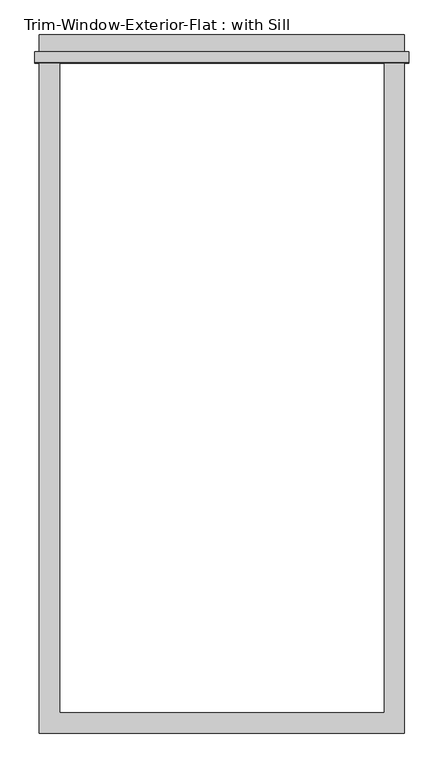
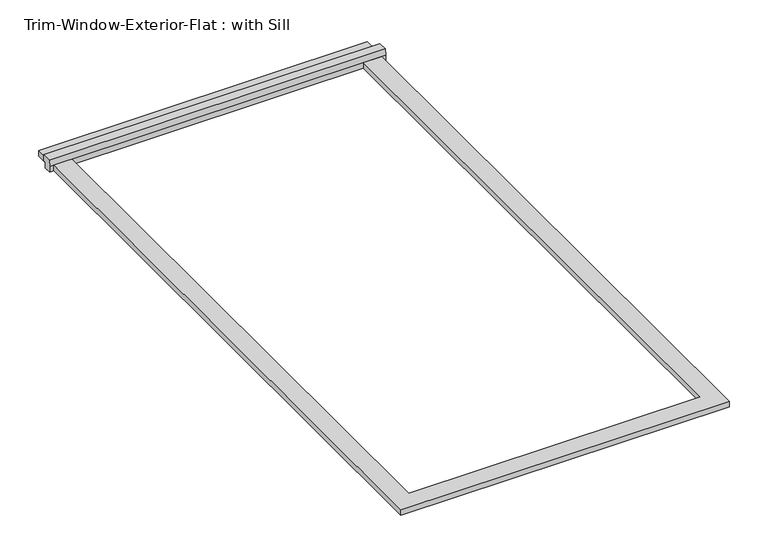
"""IFC4 building model written with IfcOpenShell, lengths in millimetres: proxy geometry, Trim-Window-Exterior-Flat : with Sill."""

from ifc_helpers import new_model, si_unit, frame, origin, origin_with_axes, place, context, project, spatial, polyline, outline, extrude, source, transform, mapped, element, save


def trim_window_exterior_flat_with_sill_0eb976c3(model_context):
    return source(origin(), model_context, "Body", "SweptSolid", [
        extrude(outline(polyline([(514.35, 1850.9823709), (-514.35, 1850.9823709), (-514.35, 1908.1323709), (514.35, 1908.1323709), (514.35, 1850.9823709)])), origin_with_axes(), (0.0, 0.0, 1.0), 19.05),
        extrude(outline(polyline([(1860.55, 38.1), (1860.55, 19.05), (1850.9823709, 19.05), (1850.9823709, 0.0), (1828.8, 0.0), (1828.8, 19.05), (1831.2580645, 38.1), (1860.55, 38.1)])), frame((-527.05, 0.0, 0.0), z_axis=(1.0, 0.0, 0.0), x_axis=(0.0, 1.0, 0.0)), (0.0, 0.0, 1.0), 1054.1),
        extrude(outline(polyline([(-514.35, -57.15), (-514.35, 1828.8), (-457.2, 1828.8), (-457.2, 0.0), (457.2, 0.0), (457.2, 1828.8), (514.35, 1828.8), (514.35, -57.15), (-514.35, -57.15)])), origin_with_axes(), (0.0, 0.0, 1.0), 19.05),
    ])


if __name__ == "__main__":
    model = new_model("IFC4")
    model_context = context("Model", 3, world=origin())
    ifc_project = project(units=[si_unit("LENGTHUNIT", "METRE", prefix="MILLI")], contexts=[model_context])
    site = spatial("IfcSite", under=ifc_project)
    building = spatial("IfcBuilding", under=site)
    placement = place(None, origin())
    trim_window_exterior_flat_with_sill_shape = trim_window_exterior_flat_with_sill_0eb976c3(model_context)
    element("IfcBuildingElementProxy", 1, Name="Trim-Window-Exterior-Flat : with Sill", ObjectType="Trim-Window-Exterior-Flat : with Sill", at=placement, inside=building, context=model_context, shape_type="MappedRepresentation", body=[
        mapped(trim_window_exterior_flat_with_sill_shape, transform((0.0, 0.0, 0.0), x_axis=(1.0, 0.0, 0.0), y_axis=(0.0, 1.0, 0.0), z_axis=(0.0, 0.0, 1.0))),
    ])
    save(model, "model.ifc")

# Revit data of these elements
# Type "Trim-Window-Exterior-Flat : with Sill"
#   Trim Width = 0' - 2 1/4"
#   Trim Thickness_Picture Frame = 0' - 1 1/4"
#   Trim Thickness_with Sill = 0' - 0 3/4"
#   Sill Thickness = 0' - 1 1/4"
#   Opening Width [instance default] = 2' - 0"
#   Opening Height [instance default] = 3' - 0"
#   Default Elevation = 4' - 0"
#   Sill = yes
#   Picture Frame = no
#   Trim Material [instance default] = none
# Element 1 (IfcBuildingElementProxy, "Trim-Window-Exterior-Flat : with Sill")
#   Opening Width = 3' - 0"
#   Opening Height = 6' - 0"
#   Trim Material = Clad - White
#   Materials on its faces: "Clad - White"
# Materials
#   "Clad - White": class "Wood", colour RGB 242 242 238, transparency 0, Cost = 0
